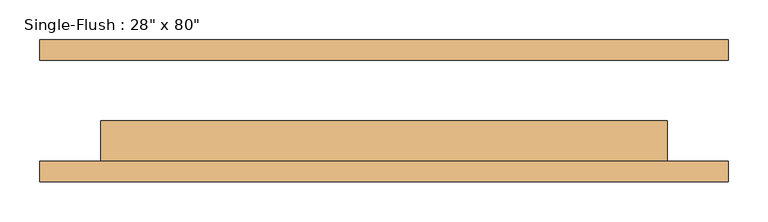
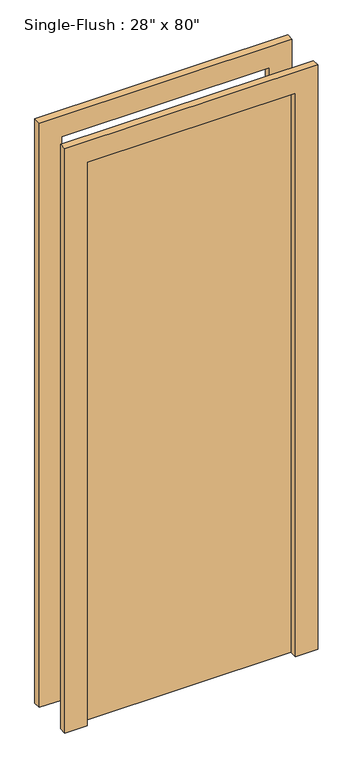
"""IFC4 building model written with IfcOpenShell, lengths in millimetres: door geometry."""

import ifcopenshell
import ifcopenshell.guid

model = None  # the IFC model being written
_history = None  # IfcOwnerHistory: only IFC2X3 demands one
_inside = {}  # id of a spatial element -> (the spatial element, [elements in it])
_under = {}  # id of a project, library or spatial element -> (it, [spatial elements below it])
_declared = {}  # id of a project -> (the project, [libraries it declares])
_typed = {}  # id of a type object -> (the type object, [elements of that type])
_made_of = {}  # id of a material, layer set ... -> (it, [elements and type objects made of it])


def new_model(schema):
    """Start an empty IFC model of exactly this schema.

    Asked for "IFC4X3", IfcOpenShell would pick the latest addendum, in which some entities
    have other attributes; the version numbers below select the first issue.
    IFC2X3 requires an IfcOwnerHistory on every rooted entity: one is made here for all.
    """
    global model, _history
    if schema == "IFC4X3":
        model = ifcopenshell.file(schema_version=(4, 3, 0, 0))
    else:
        model = ifcopenshell.file(schema=schema)
    _inside.clear()
    _under.clear()
    _declared.clear()
    _typed.clear()
    _made_of.clear()
    _history = None
    if model.schema == "IFC2X3":
        org = make("IfcOrganization", Name="unknown")
        user = make(
            "IfcPersonAndOrganization",
            ThePerson=make("IfcPerson", FamilyName="unknown"),
            TheOrganization=org,
        )
        app = make(
            "IfcApplication",
            ApplicationDeveloper=org,
            Version="unknown",
            ApplicationFullName="unknown",
            ApplicationIdentifier="unknown",
        )
        _history = make(
            "IfcOwnerHistory",
            OwningUser=user,
            OwningApplication=app,
            ChangeAction="ADDED",
            CreationDate=0,
        )
    return model


def make(cls, **values):
    """One entity of the class cls with the attributes given. An attribute that is None is left unset."""
    return model.create_entity(
        cls, **{name: value for name, value in values.items() if value is not None}
    )


def rooted(cls, **values):
    """An entity with a GlobalId (a new one), such as an element, a storey or a relation."""
    return make(cls, GlobalId=ifcopenshell.guid.new(), OwnerHistory=_history, **values)


def si_unit(unit_type, name, prefix=None):
    """IfcSIUnit, for example si_unit("LENGTHUNIT", "METRE", prefix="MILLI")."""
    return make("IfcSIUnit", UnitType=unit_type, Prefix=prefix, Name=name)


def assignment(units):
    """IfcUnitAssignment: the units of a project."""
    return None if units is None else make("IfcUnitAssignment", Units=units)


def point(xyz):
    """IfcCartesianPoint."""
    return None if xyz is None else make("IfcCartesianPoint", Coordinates=xyz)


def direction(xyz):
    """IfcDirection."""
    return None if xyz is None else make("IfcDirection", DirectionRatios=xyz)


def frame(location, z_axis=None, x_axis=None):
    """IfcAxis2Placement3D, a coordinate frame: its origin and axes. An axis left out is left unset."""
    return make(
        "IfcAxis2Placement3D",
        Location=point(location),
        Axis=direction(z_axis),
        RefDirection=direction(x_axis),
    )


def origin():
    """The frame at (0, 0, 0) with its axes left unset."""
    return frame((0.0, 0.0, 0.0))


def origin_with_axes():
    """The frame at (0, 0, 0) with the z axis (0, 0, 1) and the x axis (1, 0, 0) written out."""
    return frame((0.0, 0.0, 0.0), z_axis=(0.0, 0.0, 1.0), x_axis=(1.0, 0.0, 0.0))


def place(relative_to, where):
    """IfcLocalPlacement: puts the frame where relative to a parent placement (None: the world)."""
    return make(
        "IfcLocalPlacement", PlacementRelTo=relative_to, RelativePlacement=where
    )


def context(
    kind, dimensions, precision=None, world=None, true_north=None, identifier=None
):
    """IfcGeometricRepresentationContext, for example the 3D "Model" context."""
    return make(
        "IfcGeometricRepresentationContext",
        ContextIdentifier=identifier,
        ContextType=kind,
        CoordinateSpaceDimension=dimensions,
        Precision=precision,
        WorldCoordinateSystem=world,
        TrueNorth=true_north,
    )


def project(units=None, contexts=None):
    """IfcProject with its units and contexts."""
    return rooted(
        "IfcProject",
        Name="project",
        RepresentationContexts=contexts,
        UnitsInContext=assignment(units),
    )


def spatial(cls, under=None, at=None, **own):
    """A site, building, storey or space (cls), placed at a placement, below another one or the project."""
    s = rooted(cls, ObjectPlacement=at, **own)
    if under is not None:
        _under.setdefault(under.id(), (under, []))[1].append(s)
    return s


def polyline(points):
    """IfcPolyline through the points."""
    return make("IfcPolyline", Points=[point(p) for p in points])


def outline(outer, holes=None, kind="AREA"):
    """IfcArbitraryClosedProfileDef: a profile drawn as a closed curve; with holes, ...WithVoids."""
    if holes is None:
        return make("IfcArbitraryClosedProfileDef", ProfileType=kind, OuterCurve=outer)
    return make(
        "IfcArbitraryProfileDefWithVoids",
        ProfileType=kind,
        OuterCurve=outer,
        InnerCurves=holes,
    )


def extrude(swept, where, along, depth):
    """IfcExtrudedAreaSolid: the profile swept, set in the frame where, extruded along a direction by depth."""
    return make(
        "IfcExtrudedAreaSolid",
        SweptArea=swept,
        Position=where,
        ExtrudedDirection=direction(along),
        Depth=depth,
    )


def shape(context_of_items, identifier, shape_type, items):
    """IfcShapeRepresentation: the items that make up one representation, for example the "Body"."""
    return make(
        "IfcShapeRepresentation",
        ContextOfItems=context_of_items,
        RepresentationIdentifier=identifier,
        RepresentationType=shape_type,
        Items=items,
    )


def source(mapping_origin, context_of_items, identifier, shape_type, items):
    """IfcRepresentationMap: a shape defined once, which mapped items show again and again."""
    return make(
        "IfcRepresentationMap",
        MappingOrigin=mapping_origin,
        MappedRepresentation=shape(context_of_items, identifier, shape_type, items),
    )


def transform(
    local_origin,
    x_axis=None,
    y_axis=None,
    z_axis=None,
    scale=None,
    scale2=None,
    scale3=None,
    uniform=True,
):
    """IfcCartesianTransformationOperator3D, or its non-uniform kind. x_axis, y_axis, z_axis: its Axis1, 2, 3."""
    if uniform:
        return make(
            "IfcCartesianTransformationOperator3D",
            Axis1=direction(x_axis),
            Axis2=direction(y_axis),
            LocalOrigin=point(local_origin),
            Scale=scale,
            Axis3=direction(z_axis),
        )
    return make(
        "IfcCartesianTransformationOperator3DnonUniform",
        Axis1=direction(x_axis),
        Axis2=direction(y_axis),
        LocalOrigin=point(local_origin),
        Scale=scale,
        Axis3=direction(z_axis),
        Scale2=scale2,
        Scale3=scale3,
    )


def mapped(mapping_source, mapping_target):
    """IfcMappedItem: shows the shape of a source again, moved by a transform."""
    return make(
        "IfcMappedItem", MappingSource=mapping_source, MappingTarget=mapping_target
    )


def made_of(thing, what):
    """Note that an element or type object is made of a material, layer set ...; save() writes the relation."""
    if what is not None:
        _made_of.setdefault(what.id(), (what, []))[1].append(thing)
    return thing


def element(
    cls,
    number,
    at=None,
    inside=None,
    cuts=None,
    type_object=None,
    material=None,
    context=None,
    identifier="Body",
    shape_type=None,
    held_by="IfcProductDefinitionShape",
    body=None,
    shapes=None,
    **own,
):
    """One element of the class cls, such as IfcWall. Its Tag is "e" and its number.

    at: its placement. inside: the storey or other place that contains it. cuts: it is an
    opening in that element (IfcRelVoidsElement). A single representation is given by context,
    identifier, shape_type and body (its items); several are given by shapes. held_by: the class
    of the entity that holds the representations. save() writes the other relations.
    """
    e = rooted(cls, Tag="e%d" % number, ObjectPlacement=at, **own)
    if body is not None:
        shapes = [shape(context, identifier, shape_type, body)]
    if shapes is not None:
        e.Representation = make(held_by, Representations=shapes)
    if inside is not None:
        _inside.setdefault(inside.id(), (inside, []))[1].append(e)
    if cuts is not None:
        rooted(
            "IfcRelVoidsElement", RelatingBuildingElement=cuts, RelatedOpeningElement=e
        )
    if type_object is not None:
        _typed.setdefault(type_object.id(), (type_object, []))[1].append(e)
    return made_of(e, material)


def aggregate(whole, parts):
    """IfcRelAggregates: a whole, such as a stair, and the parts it consists of."""
    return rooted("IfcRelAggregates", RelatingObject=whole, RelatedObjects=parts)


def save(model, path):
    """Write the relations noted so far, then the file.

    IfcRelAggregates (storeys below a building ...), IfcRelContainedInSpatialStructure (elements
    in a storey), IfcRelDefinesByType, IfcRelAssociatesMaterial and IfcRelDeclares: one each for
    every whole, place, type object, material and project.
    """
    for whole, parts in _under.values():
        aggregate(whole, parts)
    for where, things in _inside.values():
        rooted(
            "IfcRelContainedInSpatialStructure",
            RelatedElements=things,
            RelatingStructure=where,
        )
    for kind, things in _typed.values():
        rooted("IfcRelDefinesByType", RelatedObjects=things, RelatingType=kind)
    for what, things in _made_of.values():
        rooted("IfcRelAssociatesMaterial", RelatedObjects=things, RelatingMaterial=what)
    for by, libraries in _declared.values():
        rooted("IfcRelDeclares", RelatingContext=by, RelatedDefinitions=libraries)
    model.write(path)


def door_c771f3ba(model_context):
    return source(origin(), model_context, "Body", "SweptSolid", [
        extrude(outline(polyline([(2108.2, -431.8), (0.0, -431.8), (0.0, -355.6), (2032.0, -355.6), (2032.0, 355.6), (0.0, 355.6), (0.0, 431.8), (2108.2, 431.8), (2108.2, -431.8)])), frame((0.0, -88.9, 0.0), z_axis=(0.0, 1.0, 0.0), x_axis=(0.0, 0.0, 1.0)), (0.0, 0.0, 1.0), 25.4),
        extrude(outline(polyline([(2108.2, 431.8), (2108.2, -431.8), (0.0, -431.8), (0.0, -355.6), (2032.0, -355.6), (2032.0, 355.6), (0.0, 355.6), (0.0, 431.8), (2108.2, 431.8)])), frame((0.0, 63.5, 0.0), z_axis=(0.0, 1.0, 0.0), x_axis=(0.0, 0.0, 1.0)), (0.0, 0.0, 1.0), 25.4),
        extrude(outline(polyline([(355.6, -12.7), (355.6, -63.5), (-355.6, -63.5), (-355.6, -12.7), (355.6, -12.7)])), origin_with_axes(), (0.0, 0.0, 1.0), 2032.0),
    ])


if __name__ == "__main__":
    model = new_model("IFC4")
    model_context = context("Model", 3, world=origin())
    ifc_project = project(units=[si_unit("LENGTHUNIT", "METRE", prefix="MILLI")], contexts=[model_context])
    site = spatial("IfcSite", under=ifc_project)
    building = spatial("IfcBuilding", under=site)
    placement = place(None, origin())
    door_shape = door_c771f3ba(model_context)
    element("IfcDoor", 1, ObjectType="Single-Flush : 28\" x 80\"", at=placement, inside=building, context=model_context, shape_type="MappedRepresentation", body=[
        mapped(door_shape, transform((0.0, 0.0, 0.0), x_axis=(1.0, 0.0, 0.0), y_axis=(0.0, 1.0, 0.0), z_axis=(0.0, 0.0, 1.0))),
    ])
    save(model, "model.ifc")

# Revit data of these elements
# Type "Single-Flush : 28\" x 80\""
#   Type Mark = "13"
#   Construction Type Id = "MDOOR"
#   Assembly Code = "C1020"
#   Analytic Construction = "Metal"
#   Thickness = 0' - 2"
#   Heat Transfer Coefficient (U) = 0.651978 BTU/(h·ft²·°F)
#   Height = 6' - 8"
#   Trim Projection Ext = 0' - 1"
#   Trim Projection Int = 0' - 1"
#   Trim Width = 0' - 3"
#   Width = 2' - 4"
#   Define Thermal Properties by = 1
#   Door Material = Door - Panel
#   Frame Material = Door - Frame
#   Visual Light Transmittance = 0
#   Solar Heat Gain Coefficient = 0
#   Function = (empty or 0)
#   Wall Closure = (empty or 0)
# Element 1 (IfcDoor, "Single-Flush : 28\" x 80\"")
#   Materials on its faces: "Door - Frame", "Door - Panel"
# Materials
#   "Door - Panel": class "Wood", colour RGB 210 159 95, transparency 0, Cost = 0
#   "Door - Frame": class "Miscellaneous", colour RGB 118 70 51, transparency 0, Cost = 0
